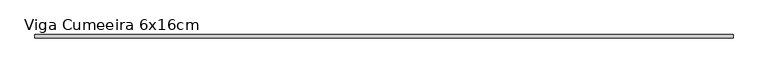
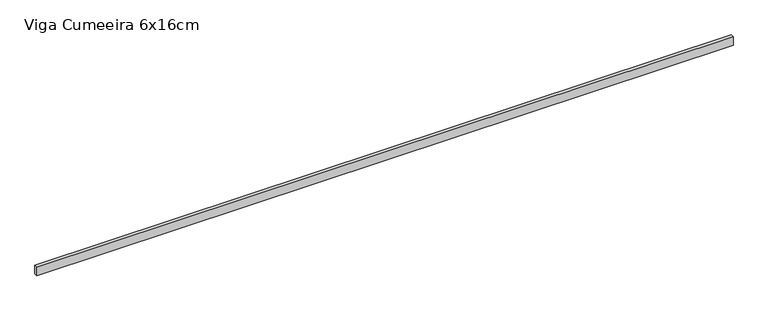
"""IFC4 building model written with IfcOpenShell, lengths in millimetres: beam geometry, Madeira de lei : Viga Cumeeira 6x16cm."""

from ifc_helpers import new_model, si_unit, frame, origin, place, context, project, spatial, polyline, outline, extrude, source, transform, mapped, element, save


def viga_cumeeira_6x16cm_b61bb166(model_context):
    return source(origin(), model_context, "Body", "SweptSolid", [
        extrude(outline(polyline([(6210.0, 30.0), (6210.0, -30.0), (-6210.0, -30.0), (-6210.0, 30.0), (6210.0, 30.0)])), frame((0.0, 0.0, -80.0), z_axis=(0.0, 0.0, 1.0), x_axis=(1.0, 0.0, 0.0)), (0.0, 0.0, 1.0), 160.0),
    ])


if __name__ == "__main__":
    model = new_model("IFC4")
    model_context = context("Model", 3, world=origin())
    ifc_project = project(units=[si_unit("LENGTHUNIT", "METRE", prefix="MILLI")], contexts=[model_context])
    site = spatial("IfcSite", under=ifc_project)
    building = spatial("IfcBuilding", under=site)
    placement = place(None, origin())
    viga_cumeeira_6x16cm_shape = viga_cumeeira_6x16cm_b61bb166(model_context)
    element("IfcBeam", 1, ObjectType="Madeira de lei : Viga Cumeeira 6x16cm", at=placement, inside=building, context=model_context, shape_type="MappedRepresentation", body=[
        mapped(viga_cumeeira_6x16cm_shape, transform((0.0, 0.0, 0.0), x_axis=(1.0, 0.0, 0.0), y_axis=(0.0, 1.0, 0.0), z_axis=(0.0, 0.0, 1.0))),
    ])
    save(model, "model.ifc")

# Revit data of these elements
# Type "Madeira de lei : Viga Cumeeira 6x16cm"
#   A = 0.02 m²
#   Length [instance default] = 1.524 m
#   b = 0.06 m
#   d = 0.16 m
#   Structural Material [instance default] = none
#   Assembly Code = ""
# Element 1 (IfcBeam, "Madeira de lei : Viga Cumeeira 6x16cm")
#   Structural Material = .MADEIRAMENTO
#   Materials on its faces: ".MADEIRAMENTO"
# Materials
#   ".MADEIRAMENTO": class ".CC_MADEIRAS", colour RGB 212 179 113, transparency 0, Cost = 0
